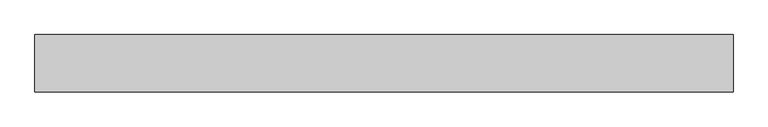
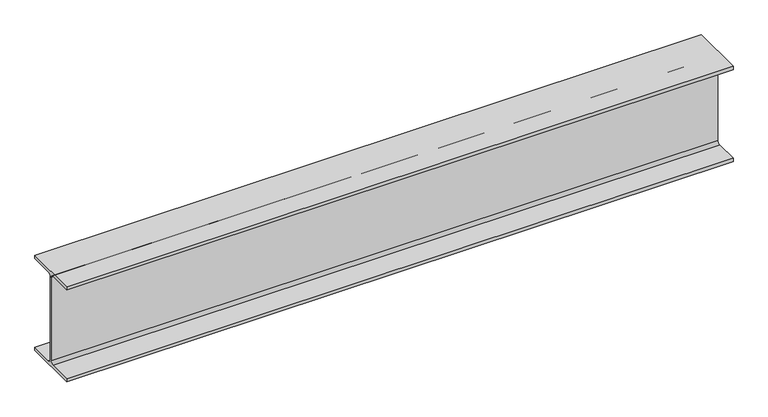
"""IFC4 building model written with IfcOpenShell, lengths in millimetres: beam geometry, Steel Beam_H-KSD3502 : H_SB_ASB_H-194x150x6x9."""

import ifcopenshell
import ifcopenshell.guid

model = None  # the IFC model being written
_history = None  # IfcOwnerHistory: only IFC2X3 demands one
_inside = {}  # id of a spatial element -> (the spatial element, [elements in it])
_under = {}  # id of a project, library or spatial element -> (it, [spatial elements below it])
_declared = {}  # id of a project -> (the project, [libraries it declares])
_typed = {}  # id of a type object -> (the type object, [elements of that type])
_made_of = {}  # id of a material, layer set ... -> (it, [elements and type objects made of it])


def new_model(schema):
    """Start an empty IFC model of exactly this schema.

    Asked for "IFC4X3", IfcOpenShell would pick the latest addendum, in which some entities
    have other attributes; the version numbers below select the first issue.
    IFC2X3 requires an IfcOwnerHistory on every rooted entity: one is made here for all.
    """
    global model, _history
    if schema == "IFC4X3":
        model = ifcopenshell.file(schema_version=(4, 3, 0, 0))
    else:
        model = ifcopenshell.file(schema=schema)
    _inside.clear()
    _under.clear()
    _declared.clear()
    _typed.clear()
    _made_of.clear()
    _history = None
    if model.schema == "IFC2X3":
        org = make("IfcOrganization", Name="unknown")
        user = make(
            "IfcPersonAndOrganization",
            ThePerson=make("IfcPerson", FamilyName="unknown"),
            TheOrganization=org,
        )
        app = make(
            "IfcApplication",
            ApplicationDeveloper=org,
            Version="unknown",
            ApplicationFullName="unknown",
            ApplicationIdentifier="unknown",
        )
        _history = make(
            "IfcOwnerHistory",
            OwningUser=user,
            OwningApplication=app,
            ChangeAction="ADDED",
            CreationDate=0,
        )
    return model


def make(cls, **values):
    """One entity of the class cls with the attributes given. An attribute that is None is left unset."""
    return model.create_entity(
        cls, **{name: value for name, value in values.items() if value is not None}
    )


def rooted(cls, **values):
    """An entity with a GlobalId (a new one), such as an element, a storey or a relation."""
    return make(cls, GlobalId=ifcopenshell.guid.new(), OwnerHistory=_history, **values)


def si_unit(unit_type, name, prefix=None):
    """IfcSIUnit, for example si_unit("LENGTHUNIT", "METRE", prefix="MILLI")."""
    return make("IfcSIUnit", UnitType=unit_type, Prefix=prefix, Name=name)


def assignment(units):
    """IfcUnitAssignment: the units of a project."""
    return None if units is None else make("IfcUnitAssignment", Units=units)


def point(xyz):
    """IfcCartesianPoint."""
    return None if xyz is None else make("IfcCartesianPoint", Coordinates=xyz)


def direction(xyz):
    """IfcDirection."""
    return None if xyz is None else make("IfcDirection", DirectionRatios=xyz)


def frame(location, z_axis=None, x_axis=None):
    """IfcAxis2Placement3D, a coordinate frame: its origin and axes. An axis left out is left unset."""
    return make(
        "IfcAxis2Placement3D",
        Location=point(location),
        Axis=direction(z_axis),
        RefDirection=direction(x_axis),
    )


def frame_2d(location, x_axis=None):
    """IfcAxis2Placement2D, a coordinate frame in the plane: its origin and x axis."""
    return make(
        "IfcAxis2Placement2D", Location=point(location), RefDirection=direction(x_axis)
    )


def origin():
    """The frame at (0, 0, 0) with its axes left unset."""
    return frame((0.0, 0.0, 0.0))


def place(relative_to, where):
    """IfcLocalPlacement: puts the frame where relative to a parent placement (None: the world)."""
    return make(
        "IfcLocalPlacement", PlacementRelTo=relative_to, RelativePlacement=where
    )


def context(
    kind, dimensions, precision=None, world=None, true_north=None, identifier=None
):
    """IfcGeometricRepresentationContext, for example the 3D "Model" context."""
    return make(
        "IfcGeometricRepresentationContext",
        ContextIdentifier=identifier,
        ContextType=kind,
        CoordinateSpaceDimension=dimensions,
        Precision=precision,
        WorldCoordinateSystem=world,
        TrueNorth=true_north,
    )


def project(units=None, contexts=None):
    """IfcProject with its units and contexts."""
    return rooted(
        "IfcProject",
        Name="project",
        RepresentationContexts=contexts,
        UnitsInContext=assignment(units),
    )


def spatial(cls, under=None, at=None, **own):
    """A site, building, storey or space (cls), placed at a placement, below another one or the project."""
    s = rooted(cls, ObjectPlacement=at, **own)
    if under is not None:
        _under.setdefault(under.id(), (under, []))[1].append(s)
    return s


def polyline(points):
    """IfcPolyline through the points."""
    return make("IfcPolyline", Points=[point(p) for p in points])


def circle_curve(where, radius):
    """IfcCircle in the frame where."""
    return make("IfcCircle", Position=where, Radius=radius)


def trimmed(basis, trim1, trim2, sense, master):
    """IfcTrimmedCurve: the piece of a basis curve between two trims."""
    return make(
        "IfcTrimmedCurve",
        BasisCurve=basis,
        Trim1=trim1,
        Trim2=trim2,
        SenseAgreement=sense,
        MasterRepresentation=master,
    )


def segment(curve, same_sense, transition):
    """IfcCompositeCurveSegment."""
    return make(
        "IfcCompositeCurveSegment",
        Transition=transition,
        SameSense=same_sense,
        ParentCurve=curve,
    )


def composite_curve(segments, self_intersect=None):
    """IfcCompositeCurve: segments joined end to end."""
    return make("IfcCompositeCurve", Segments=segments, SelfIntersect=self_intersect)


def outline(outer, holes=None, kind="AREA"):
    """IfcArbitraryClosedProfileDef: a profile drawn as a closed curve; with holes, ...WithVoids."""
    if holes is None:
        return make("IfcArbitraryClosedProfileDef", ProfileType=kind, OuterCurve=outer)
    return make(
        "IfcArbitraryProfileDefWithVoids",
        ProfileType=kind,
        OuterCurve=outer,
        InnerCurves=holes,
    )


def extrude(swept, where, along, depth):
    """IfcExtrudedAreaSolid: the profile swept, set in the frame where, extruded along a direction by depth."""
    return make(
        "IfcExtrudedAreaSolid",
        SweptArea=swept,
        Position=where,
        ExtrudedDirection=direction(along),
        Depth=depth,
    )


def shape(context_of_items, identifier, shape_type, items):
    """IfcShapeRepresentation: the items that make up one representation, for example the "Body"."""
    return make(
        "IfcShapeRepresentation",
        ContextOfItems=context_of_items,
        RepresentationIdentifier=identifier,
        RepresentationType=shape_type,
        Items=items,
    )


def source(mapping_origin, context_of_items, identifier, shape_type, items):
    """IfcRepresentationMap: a shape defined once, which mapped items show again and again."""
    return make(
        "IfcRepresentationMap",
        MappingOrigin=mapping_origin,
        MappedRepresentation=shape(context_of_items, identifier, shape_type, items),
    )


def transform(
    local_origin,
    x_axis=None,
    y_axis=None,
    z_axis=None,
    scale=None,
    scale2=None,
    scale3=None,
    uniform=True,
):
    """IfcCartesianTransformationOperator3D, or its non-uniform kind. x_axis, y_axis, z_axis: its Axis1, 2, 3."""
    if uniform:
        return make(
            "IfcCartesianTransformationOperator3D",
            Axis1=direction(x_axis),
            Axis2=direction(y_axis),
            LocalOrigin=point(local_origin),
            Scale=scale,
            Axis3=direction(z_axis),
        )
    return make(
        "IfcCartesianTransformationOperator3DnonUniform",
        Axis1=direction(x_axis),
        Axis2=direction(y_axis),
        LocalOrigin=point(local_origin),
        Scale=scale,
        Axis3=direction(z_axis),
        Scale2=scale2,
        Scale3=scale3,
    )


def mapped(mapping_source, mapping_target):
    """IfcMappedItem: shows the shape of a source again, moved by a transform."""
    return make(
        "IfcMappedItem", MappingSource=mapping_source, MappingTarget=mapping_target
    )


def made_of(thing, what):
    """Note that an element or type object is made of a material, layer set ...; save() writes the relation."""
    if what is not None:
        _made_of.setdefault(what.id(), (what, []))[1].append(thing)
    return thing


def element(
    cls,
    number,
    at=None,
    inside=None,
    cuts=None,
    type_object=None,
    material=None,
    context=None,
    identifier="Body",
    shape_type=None,
    held_by="IfcProductDefinitionShape",
    body=None,
    shapes=None,
    **own,
):
    """One element of the class cls, such as IfcWall. Its Tag is "e" and its number.

    at: its placement. inside: the storey or other place that contains it. cuts: it is an
    opening in that element (IfcRelVoidsElement). A single representation is given by context,
    identifier, shape_type and body (its items); several are given by shapes. held_by: the class
    of the entity that holds the representations. save() writes the other relations.
    """
    e = rooted(cls, Tag="e%d" % number, ObjectPlacement=at, **own)
    if body is not None:
        shapes = [shape(context, identifier, shape_type, body)]
    if shapes is not None:
        e.Representation = make(held_by, Representations=shapes)
    if inside is not None:
        _inside.setdefault(inside.id(), (inside, []))[1].append(e)
    if cuts is not None:
        rooted(
            "IfcRelVoidsElement", RelatingBuildingElement=cuts, RelatedOpeningElement=e
        )
    if type_object is not None:
        _typed.setdefault(type_object.id(), (type_object, []))[1].append(e)
    return made_of(e, material)


def aggregate(whole, parts):
    """IfcRelAggregates: a whole, such as a stair, and the parts it consists of."""
    return rooted("IfcRelAggregates", RelatingObject=whole, RelatedObjects=parts)


def save(model, path):
    """Write the relations noted so far, then the file.

    IfcRelAggregates (storeys below a building ...), IfcRelContainedInSpatialStructure (elements
    in a storey), IfcRelDefinesByType, IfcRelAssociatesMaterial and IfcRelDeclares: one each for
    every whole, place, type object, material and project.
    """
    for whole, parts in _under.values():
        aggregate(whole, parts)
    for where, things in _inside.values():
        rooted(
            "IfcRelContainedInSpatialStructure",
            RelatedElements=things,
            RelatingStructure=where,
        )
    for kind, things in _typed.values():
        rooted("IfcRelDefinesByType", RelatedObjects=things, RelatingType=kind)
    for what, things in _made_of.values():
        rooted("IfcRelAssociatesMaterial", RelatedObjects=things, RelatingMaterial=what)
    for by, libraries in _declared.values():
        rooted("IfcRelDeclares", RelatingContext=by, RelatedDefinitions=libraries)
    model.write(path)


def beam_e603d65a(model_context):
    return source(origin(), model_context, "Body", "SweptSolid", [
        extrude(outline(composite_curve([segment(polyline([(-82.5, -141.5), (-11.9, -141.5)]), True, "CONTINUOUS"), segment(trimmed(circle_curve(frame_2d((-11.9, -132.6)), 8.9), [point((-11.9, -141.5))], [point((-3.0, -132.6))], True, "CARTESIAN"), True, "CONTINUOUS"), segment(polyline([(-3.0, -132.6), (-3.0, 132.6)]), True, "CONTINUOUS"), segment(trimmed(circle_curve(frame_2d((-11.9, 132.6)), 8.9), [point((-3.0, 132.6))], [point((-11.9, 141.5))], True, "CARTESIAN"), True, "CONTINUOUS"), segment(polyline([(-11.9, 141.5), (-82.5, 141.5), (-82.5, 151.7), (82.5, 151.7), (82.5, 141.5), (11.9, 141.5)]), True, "CONTINUOUS"), segment(trimmed(circle_curve(frame_2d((11.9, 132.6)), 8.9), [point((11.9, 141.5))], [point((3.0, 132.6))], True, "CARTESIAN"), True, "CONTINUOUS"), segment(polyline([(3.0, 132.6), (3.0, -132.6)]), True, "CONTINUOUS"), segment(trimmed(circle_curve(frame_2d((11.9, -132.6)), 8.9), [point((3.0, -132.6))], [point((11.9, -141.5))], True, "CARTESIAN"), True, "CONTINUOUS"), segment(polyline([(11.9, -141.5), (82.5, -141.5), (82.5, -151.7), (-82.5, -151.7), (-82.5, -141.5)]), True, "CONTINUOUS")], self_intersect=False)), frame((-1171.2564634, 0.0, 0.0), z_axis=(1.0, 0.0, 0.0), x_axis=(0.0, 1.0, 0.0)), (0.0, 0.0, 1.0), 2006.3303739),
    ])


if __name__ == "__main__":
    model = new_model("IFC4")
    model_context = context("Model", 3, world=origin())
    ifc_project = project(units=[si_unit("LENGTHUNIT", "METRE", prefix="MILLI")], contexts=[model_context])
    site = spatial("IfcSite", under=ifc_project)
    building = spatial("IfcBuilding", under=site)
    placement = place(None, origin())
    beam_shape = beam_e603d65a(model_context)
    element("IfcBeam", 1, ObjectType="Steel Beam_H-KSD3502 : H_SB_ASB_H-194x150x6x9", at=placement, inside=building, context=model_context, shape_type="MappedRepresentation", body=[
        mapped(beam_shape, transform((0.0, 0.0, 0.0), x_axis=(1.0, 0.0, 0.0), y_axis=(0.0, 1.0, 0.0), z_axis=(0.0, 0.0, 1.0))),
    ])
    save(model, "model.ifc")

# Revit data of these elements
# Type "Steel Beam_H-KSD3502 : H_SB_ASB_H-194x150x6x9"
#   Width = 15.0 cm
#   Web Thickness = 0.6 cm
#   Web Fillet = 1.3 cm
#   Warping Constant = 43316.0 cm⁶
#   Torsional Moment of Inertia = 8.622 cm⁴
#   Torsional Modulus = 1.0 cm³
#   Section Area = 39.01 cm²
#   Plastic Modulus weak axis = 104.0 cm³
#   Plastic Modulus strong axis = 309.0 cm³
#   Perimeter = 0.95 m²/m
#   Nominal Weight = 30.60 kgf/m
#   Moment of Inertia weak axis = 507.00 cm⁴
#   Moment of Inertia strong axis = 2690.00 cm⁴
#   Height = 19.4 cm
#   Flange Thickness = 0.9 cm
#   Elastic Modulus weak axis = 67.6 cm³
#   Elastic Modulus strong axis = 277.0 cm³
#   Centroid Vertical = 9.7 cm
#   Centroid Horizontal = 7.5 cm
#   Length [instance default] = 1.5240 m
#   Structural Material [instance default] = Steel, 45-345
#   Assembly Code = ""
# Element 1 (IfcBeam, "Steel Beam_H-KSD3502 : H_SB_ASB_H-194x150x6x9")
#   Structural Material = none
# Materials
#   "Steel, 45-345": class "Metal", colour RGB 189 187 185, transparency 0, Description = "Steel 345 MPa", Cost = 0
